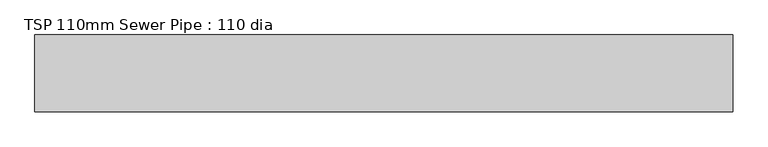
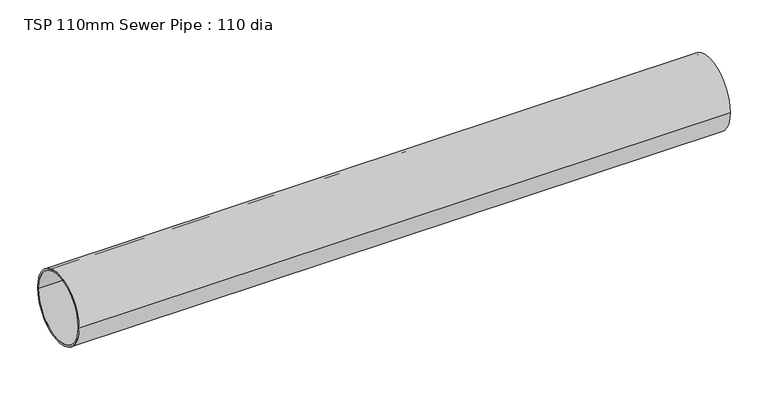
"""IFC4 building model written with IfcOpenShell, lengths in millimetres: flow terminal geometry, TSP 110mm Sewer Pipe : 110 dia."""

from ifc_helpers import new_model, si_unit, point, frame, origin, origin_2d, place, context, project, spatial, circle_curve, trimmed, segment, composite_curve, outline, extrude, source, transform, mapped, element, save


def tsp_110mm_sewer_pipe_110_dia_338e20ea(model_context):
    return source(origin(), model_context, "Body", "SweptSolid", [
        extrude(outline(composite_curve([segment(trimmed(circle_curve(origin_2d(), 55.0), [point((-55.0, 0.0))], [point((55.0, 0.0))], False, "CARTESIAN"), True, "CONTINUOUS"), segment(trimmed(circle_curve(origin_2d(), 55.0), [point((55.0, 0.0))], [point((-55.0, 0.0))], False, "CARTESIAN"), True, "CONTINUOUS")], self_intersect=False), holes=[composite_curve([segment(trimmed(circle_curve(origin_2d(), 52.0), [point((-52.0, 0.0))], [point((52.0, 0.0))], True, "CARTESIAN"), True, "CONTINUOUS"), segment(trimmed(circle_curve(origin_2d(), 52.0), [point((52.0, 0.0))], [point((-52.0, 0.0))], True, "CARTESIAN"), True, "CONTINUOUS")], self_intersect=False)]), frame((0.0, 0.0, 0.0), z_axis=(1.0, 0.0, 0.0), x_axis=(0.0, 1.0, 0.0)), (0.0, 0.0, 1.0), 1000.0),
    ])


if __name__ == "__main__":
    model = new_model("IFC4")
    model_context = context("Model", 3, world=origin())
    ifc_project = project(units=[si_unit("LENGTHUNIT", "METRE", prefix="MILLI")], contexts=[model_context])
    site = spatial("IfcSite", under=ifc_project)
    building = spatial("IfcBuilding", under=site)
    placement = place(None, origin())
    tsp_110mm_sewer_pipe_110_dia_shape = tsp_110mm_sewer_pipe_110_dia_338e20ea(model_context)
    element("IfcFlowTerminal", 1, ObjectType="TSP 110mm Sewer Pipe : 110 dia", at=placement, inside=building, context=model_context, shape_type="MappedRepresentation", body=[
        mapped(tsp_110mm_sewer_pipe_110_dia_shape, transform((0.0, 0.0, 0.0), x_axis=(1.0, 0.0, 0.0), y_axis=(0.0, 1.0, 0.0), z_axis=(0.0, 0.0, 1.0))),
    ])
    save(model, "model.ifc")

# Revit data of these elements
# Type "TSP 110mm Sewer Pipe : 110 dia"
#   Model = "TSP_110SWB"
#   Model = "TSP_110SWB"
#   Pipe length [instance default] = 1200 mm
#   Pipe dia = 110 mm
#   built-in parameter 1001306 [instance default] = 3.93701 (stored number, unit not read)
#   Default Elevation = 0
# Element 1 (IfcFlowTerminal, "TSP 110mm Sewer Pipe : 110 dia")
#   Pipe length = 1000 mm
#   built-in parameter 1001306 = 3.28084 (stored number, unit not read)
#   Materials on its faces: "Laminate, Brown, Matte"
# Materials
#   "Laminate, Brown, Matte": class "Plastic", colour RGB 128 64 0, transparency 0, Description = "Plastic Laminate - Red, Matte", Cost = 0
